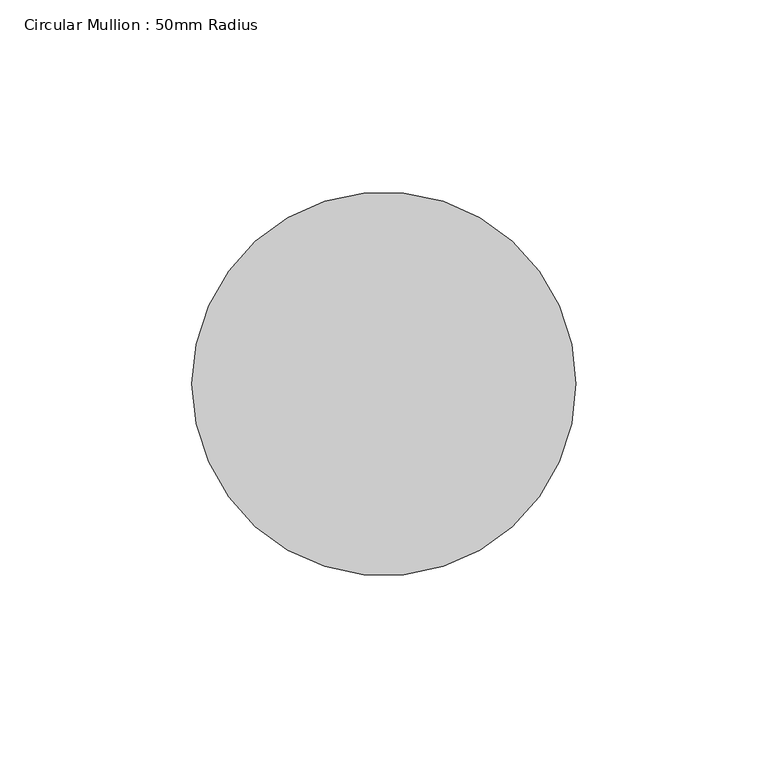
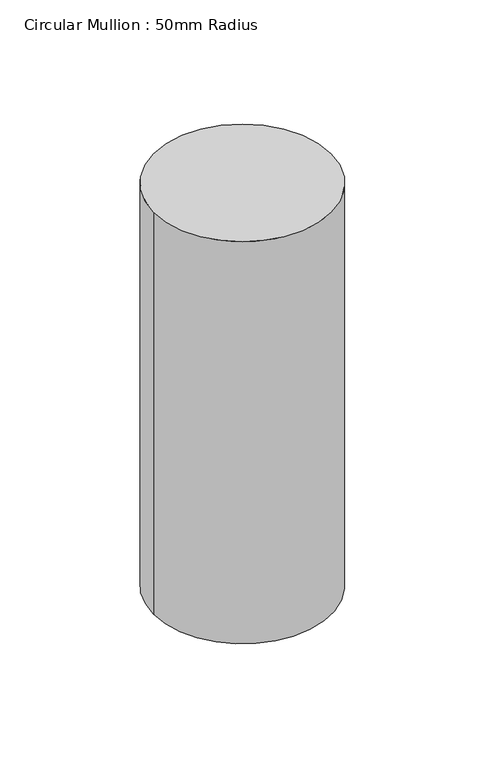
"""IFC4 building model written with IfcOpenShell, lengths in millimetres: member geometry, Circular Mullion : 50mm Radius."""

from ifc_helpers import new_model, si_unit, point, frame, origin, origin_2d, place, context, project, spatial, circle_curve, trimmed, segment, composite_curve, outline, extrude, source, transform, mapped, element, save


def circular_mullion_50mm_radius_03466230(model_context):
    return source(origin(), model_context, "Body", "SweptSolid", [
        extrude(outline(composite_curve([segment(trimmed(circle_curve(origin_2d(), 50.0), [point((50.0, 0.0))], [point((-50.0, 0.0))], False, "CARTESIAN"), True, "CONTINUOUS"), segment(trimmed(circle_curve(origin_2d(), 50.0), [point((-50.0, 0.0))], [point((50.0, 0.0))], False, "CARTESIAN"), True, "CONTINUOUS")], self_intersect=False)), frame((0.0, 0.0, -239.354624), z_axis=(0.0, 0.0, 1.0), x_axis=(1.0, 0.0, 0.0)), (0.0, 0.0, 1.0), 239.354624),
    ])


if __name__ == "__main__":
    model = new_model("IFC4")
    model_context = context("Model", 3, world=origin())
    ifc_project = project(units=[si_unit("LENGTHUNIT", "METRE", prefix="MILLI")], contexts=[model_context])
    site = spatial("IfcSite", under=ifc_project)
    building = spatial("IfcBuilding", under=site)
    placement = place(None, origin())
    circular_mullion_50mm_radius_shape = circular_mullion_50mm_radius_03466230(model_context)
    element("IfcMember", 1, ObjectType="Circular Mullion : 50mm Radius", at=placement, inside=building, context=model_context, shape_type="MappedRepresentation", body=[
        mapped(circular_mullion_50mm_radius_shape, transform((0.0, 0.0, 0.0), x_axis=(1.0, 0.0, 0.0), y_axis=(0.0, 1.0, 0.0), z_axis=(0.0, 0.0, 1.0))),
    ])
    save(model, "model.ifc")

# Revit data of these elements
# Type "Circular Mullion : 50mm Radius"
#   built-in parameter 1007350 = 0.164042 (stored number, unit not read)
# Element 1 (IfcMember, "Circular Mullion : 50mm Radius")
#   Materials on its faces: "Aluminium"
# Materials
#   "Aluminium": class "Metal", colour RGB 247 247 247, transparency 0, Description = "Aluminium 6061", Cost = 0
